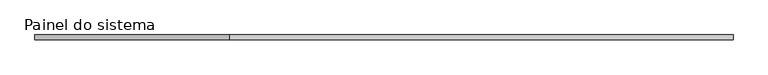
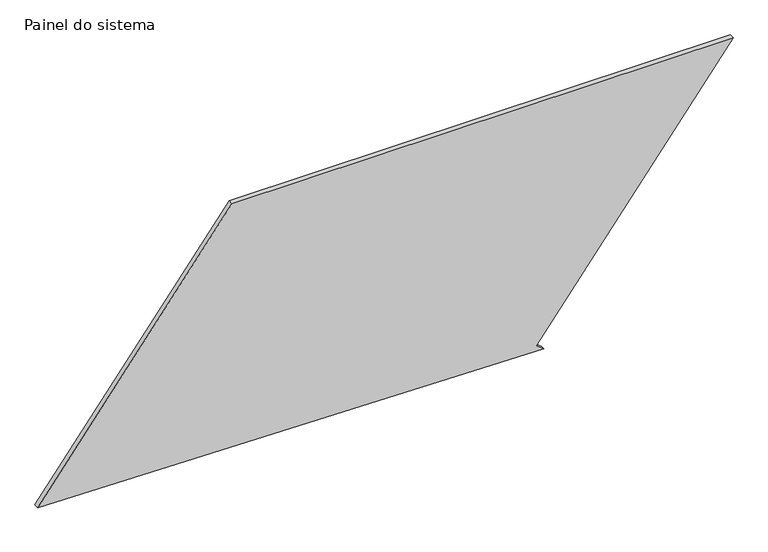
"""IFC4 building model written with IfcOpenShell, lengths in millimetres: plate geometry, Painel do sistema : Envidraçado."""

from ifc_helpers import new_model, si_unit, frame, origin, place, context, project, spatial, polyline, outline, extrude, source, transform, mapped, element, save


def painel_do_sistema_7c3fc5f4(model_context):
    return source(origin(), model_context, "Body", "SweptSolid", [
        extrude(outline(polyline([(0.0, 821.1542355), (30.4126703, 781.4670904), (1362.6283677, 1802.357777), (1362.6283677, -795.2784227), (48.4358279, -1802.357777), (0.0, 821.1542355)])), frame((0.0, 24.5, 0.0), z_axis=(0.0, 1.0, 0.0), x_axis=(0.0, 0.0, 1.0)), (0.0, 0.0, 1.0), 25.0),
    ])


if __name__ == "__main__":
    model = new_model("IFC4")
    model_context = context("Model", 3, world=origin())
    ifc_project = project(units=[si_unit("LENGTHUNIT", "METRE", prefix="MILLI")], contexts=[model_context])
    site = spatial("IfcSite", under=ifc_project)
    building = spatial("IfcBuilding", under=site)
    placement = place(None, origin())
    painel_do_sistema_shape = painel_do_sistema_7c3fc5f4(model_context)
    element("IfcPlate", 1, ObjectType="Painel do sistema : Envidraçado", at=placement, inside=building, context=model_context, shape_type="MappedRepresentation", body=[
        mapped(painel_do_sistema_shape, transform((0.0, 0.0, 0.0), x_axis=(1.0, 0.0, 0.0), y_axis=(0.0, 1.0, 0.0), z_axis=(0.0, 0.0, 1.0))),
    ])
    save(model, "model.ifc")

# Revit data of these elements
# Type "Painel do sistema : Envidraçado"
#   Construction Type Id = "GSP4R"
#   Analytic Construction = "Vidraça única Pilkington 1/8 pol"
#   Visual Light Transmittance = 0.9
#   Solar Heat Gain Coefficient = 0.86
#   Heat Transfer Coefficient (U) = 6.7069 W/(m²·K)
# Element 1 (IfcPlate, "Painel do sistema : Envidraçado")
#   Materials on its faces: "Vidro"
# Materials
#   "Vidro": class "Vidro", colour RGB 0 128 192, transparency 0.9, Description = "Vidro de sílica", Cost = 0
